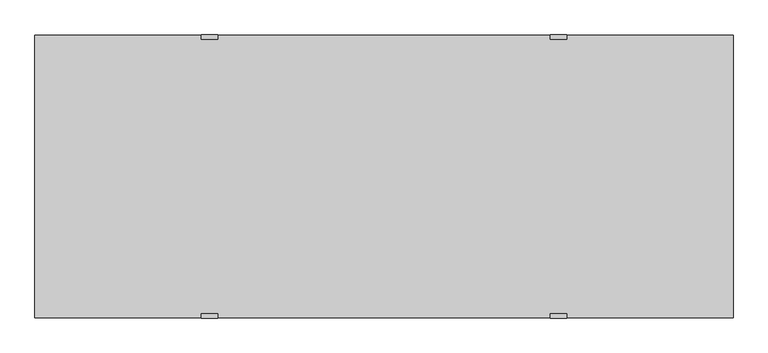
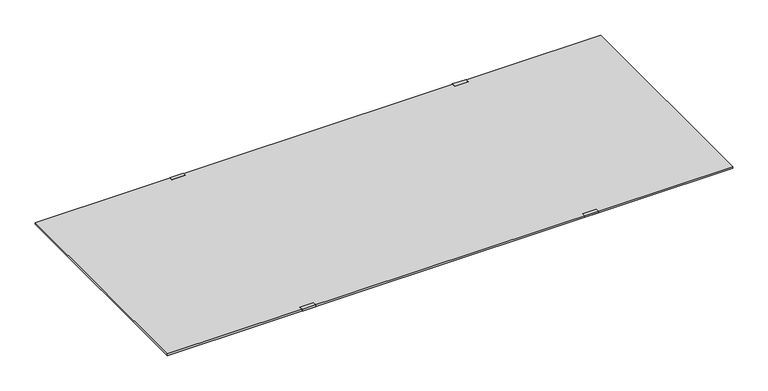
"""IFC4 building model written with IfcOpenShell, lengths in millimetres: proxy geometry."""

from ifc_helpers import new_model, si_unit, frame, origin, origin_with_axes, place, context, project, spatial, polyline, outline, extrude, source, transform, mapped, element, save


def specialty_equipment_ab541c14(model_context):
    return source(origin(), model_context, "Body", "SweptSolid", [
        extrude(outline(polyline([(431.8, 6.35), (419.1, 6.35), (419.1, 7.14375), (432.59375, 7.14375), (432.59375, 0.0), (431.8, 0.0), (431.8, 6.35)])), frame((508.0, 0.0, 0.0), z_axis=(1.0, 0.0, 0.0), x_axis=(0.0, 1.0, 0.0)), (0.0, 0.0, 1.0), 50.8),
        extrude(outline(polyline([(431.8, 6.35), (419.1, 6.35), (419.1, 7.14375), (432.59375, 7.14375), (432.59375, 0.0), (431.8, 0.0), (431.8, 6.35)])), frame((-558.8, 0.0, 0.0), z_axis=(1.0, 0.0, 0.0), x_axis=(0.0, 1.0, 0.0)), (0.0, 0.0, 1.0), 50.8),
        extrude(outline(polyline([(-431.8, 6.35), (-431.8, 0.0), (-432.59375, 0.0), (-432.59375, 7.14375), (-419.1, 7.14375), (-419.1, 6.35), (-431.8, 6.35)])), frame((508.0, 0.0, 0.0), z_axis=(1.0, 0.0, 0.0), x_axis=(0.0, 1.0, 0.0)), (0.0, 0.0, 1.0), 50.8),
        extrude(outline(polyline([(-431.8, 6.35), (-431.8, 0.0), (-432.59375, 0.0), (-432.59375, 7.14375), (-419.1, 7.14375), (-419.1, 6.35), (-431.8, 6.35)])), frame((-558.8, 0.0, 0.0), z_axis=(1.0, 0.0, 0.0), x_axis=(0.0, 1.0, 0.0)), (0.0, 0.0, 1.0), 50.8),
        extrude(outline(polyline([(1066.8, -431.8), (-1066.8, -431.8), (-1066.8, 431.8), (1066.8, 431.8), (1066.8, -431.8)])), origin_with_axes(), (0.0, 0.0, 1.0), 6.35),
    ])


if __name__ == "__main__":
    model = new_model("IFC4")
    model_context = context("Model", 3, world=origin())
    ifc_project = project(units=[si_unit("LENGTHUNIT", "METRE", prefix="MILLI")], contexts=[model_context])
    site = spatial("IfcSite", under=ifc_project)
    building = spatial("IfcBuilding", under=site)
    placement = place(None, origin())
    specialty_equipment_shape = specialty_equipment_ab541c14(model_context)
    element("IfcBuildingElementProxy", 1, Name="Bradley-Washroom_Accessories-Mirrors-747_Standard : 84\" x 36\" + BradEX", ObjectType="Bradley-Washroom_Accessories-Mirrors-747_Standard : 84\" x 36\" + BradEX", at=placement, inside=building, context=model_context, shape_type="MappedRepresentation", body=[
        mapped(specialty_equipment_shape, transform((0.0, 0.0, 0.0), x_axis=(1.0, 0.0, 0.0), y_axis=(0.0, 1.0, 0.0), z_axis=(0.0, 0.0, 1.0))),
    ])
    save(model, "model.ifc")

# Revit data of these elements
# Type "Bradley-Washroom_Accessories-Mirrors-747_Standard : 84\" x 36\" + BradEX"
#   Keynote = "M08831300.01"
#   Warranty Information = "Complete unit, excepting mirrors warranted for one year.\r\n Stainless steel mirror frames for fifteen years.\r\n Plate glass mirrors for fifteen years.\r\n This warranty does not cover installation or any other labor charges and does not apply to any units,\r\n which have been damaged by accident, abuse, improper installation, improper maintenance, or altered in any way."
#   Version = "1.0"
#   URL = "http://www.bradleycorp.com/"
#   Type Comments = "BradEX 1/4\" Float Glass Mirror"
#   OmniClass Title = "Mirrors"
#   OmniClass Code = "23.40.95.17.17"
#   Modeling Code = ""
#   Model = "747-024360"
#   MasterFormat Title = "Commercial Toilet Accessories"
#   MasterFormat Number = "10 28 13. 13"
#   Manufacturer = "Bradley Corporation"
#   Industry Standards = "ASTM C 1036"
#   Fire Rating = "n/a"
#   Description = "Frameless Mirror, Clip Fasteners, 24 by 36 inches"
#   Copyright = "This Model Data is Property of Bradley Corporation"
#   Buy American Act = "Yes"
#   Assembly Code = "C1030900"
#   ADA Compliant = "Yes"
#   Width = 7' - 0"
#   Height = 2' - 10"
#   Fastener Placement = 1' - 9"
#   Depth = 0' - 0 1/4"
#   Default Elevation = 3' - 4"
#   Reflective Material = Glass - Bradley Corp - BradEX - Polished Float Mirror
#   Frame Material = Bradley Corp Stainless Steel - Satin
# Element 1 (IfcBuildingElementProxy, "Bradley-Washroom_Accessories-Mirrors-747_Standard : 84\" x 36\" + BradEX")
#   Materials on its faces: "Bradley Corp Stainless Steel - Satin", "Glass - Bradley Corp - BradEX - Polished Float Mirror"
# Materials
#   "Glass - Bradley Corp - BradEX - Polished Float Mirror": class "Glass", colour RGB 221 230 232, transparency 0, Manufacturer = "Bradley Corporation", URL = "www.bradleycorp.com", Description = "Stainless Steel - Satin Finish", Cost = 0
#   "Bradley Corp Stainless Steel - Satin": class "Metal", colour RGB 189 187 185, transparency 0, Manufacturer = "Bradley Corporation", URL = "www.bradleycorp.com", Description = "Stainless Steel - Satin Finish", Cost = 0
